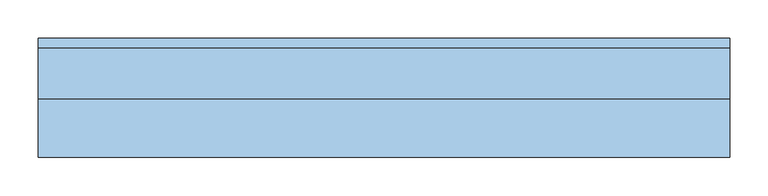
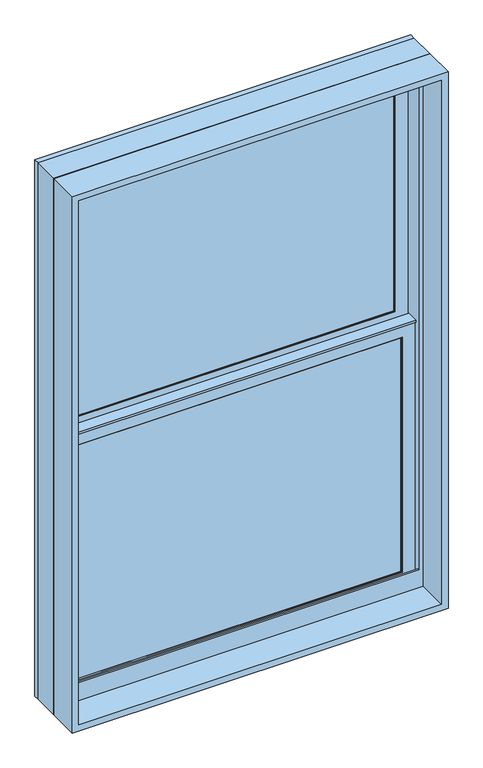
"""IFC4 building model written with IfcOpenShell, lengths in millimetres: window geometry, Window-Double_Hung-Marvin-Essential : ESDH3046."""

from ifc_helpers import new_model, si_unit, frame, origin, place, context, project, spatial, polyline, outline, extrude, faceted_brep, source, transform, mapped, element, save


def window_b4728585(model_context):
    return source(origin(), model_context, "Body", "SolidModel", [
        extrude(outline(polyline([(140.7583333, 20.6375), (140.7583333, 15.875), (121.7083333, 15.875), (121.7083333, 20.6375), (140.7583333, 20.6375)])), frame((0.0, 0.0, 1136.65), z_axis=(0.0, 0.0, 1.0), x_axis=(1.0, 0.0, 0.0)), (0.0, 0.0, 1.0), 603.25),
        extrude(outline(polyline([(-121.7083333, 20.6375), (-121.7083333, 15.875), (-140.7583333, 15.875), (-140.7583333, 20.6375), (-121.7083333, 20.6375)])), frame((0.0, 0.0, 1136.65), z_axis=(0.0, 0.0, 1.0), x_axis=(1.0, 0.0, 0.0)), (0.0, 0.0, 1.0), 603.25),
        extrude(outline(polyline([(393.7, 20.6375), (393.7, 15.875), (-393.7, 15.875), (-393.7, 20.6375), (393.7, 20.6375)])), frame((0.0, 0.0, 1428.75), z_axis=(0.0, 0.0, 1.0), x_axis=(1.0, 0.0, 0.0)), (0.0, 0.0, 1.0), 19.05),
        extrude(outline(polyline([(-140.7583333, 46.83125), (-140.7583333, 51.59375), (-121.7083333, 51.59375), (-121.7083333, 46.83125), (-140.7583333, 46.83125)])), frame((0.0, 0.0, 1778.0), z_axis=(0.0, 0.0, 1.0), x_axis=(1.0, 0.0, 0.0)), (0.0, 0.0, 1.0), 603.25),
        extrude(outline(polyline([(121.7083333, 46.83125), (121.7083333, 51.59375), (140.7583333, 51.59375), (140.7583333, 46.83125), (121.7083333, 46.83125)])), frame((0.0, 0.0, 1778.0), z_axis=(0.0, 0.0, 1.0), x_axis=(1.0, 0.0, 0.0)), (0.0, 0.0, 1.0), 603.25),
        extrude(outline(polyline([(-393.7, 46.83125), (-393.7, 51.59375), (393.7, 51.59375), (393.7, 46.83125), (-393.7, 46.83125)])), frame((0.0, 0.0, 2070.1), z_axis=(0.0, 0.0, 1.0), x_axis=(1.0, 0.0, 0.0)), (0.0, 0.0, 1.0), 19.05),
        extrude(outline(polyline([(140.7583333, 20.6375), (121.7083333, 20.6375), (121.7083333, 25.4), (140.7583333, 25.4), (140.7583333, 20.6375)])), frame((0.0, 0.0, 1136.65), z_axis=(0.0, 0.0, 1.0), x_axis=(1.0, 0.0, 0.0)), (0.0, 0.0, 1.0), 603.25),
        extrude(outline(polyline([(-121.7083333, 20.6375), (-140.7583333, 20.6375), (-140.7583333, 25.4), (-121.7083333, 25.4), (-121.7083333, 20.6375)])), frame((0.0, 0.0, 1136.65), z_axis=(0.0, 0.0, 1.0), x_axis=(1.0, 0.0, 0.0)), (0.0, 0.0, 1.0), 603.25),
        extrude(outline(polyline([(393.7, 20.6375), (-393.7, 20.6375), (-393.7, 25.4), (393.7, 25.4), (393.7, 20.6375)])), frame((0.0, 0.0, 1428.75), z_axis=(0.0, 0.0, 1.0), x_axis=(1.0, 0.0, 0.0)), (0.0, 0.0, 1.0), 19.05),
        extrude(outline(polyline([(-140.7583333, 56.35625), (-121.7083333, 56.35625), (-121.7083333, 51.59375), (-140.7583333, 51.59375), (-140.7583333, 56.35625)])), frame((0.0, 0.0, 1778.0), z_axis=(0.0, 0.0, 1.0), x_axis=(1.0, 0.0, 0.0)), (0.0, 0.0, 1.0), 603.25),
        extrude(outline(polyline([(121.7083333, 56.35625), (140.7583333, 56.35625), (140.7583333, 51.59375), (121.7083333, 51.59375), (121.7083333, 56.35625)])), frame((0.0, 0.0, 1778.0), z_axis=(0.0, 0.0, 1.0), x_axis=(1.0, 0.0, 0.0)), (0.0, 0.0, 1.0), 603.25),
        extrude(outline(polyline([(-393.7, 56.35625), (393.7, 56.35625), (393.7, 51.59375), (-393.7, 51.59375), (-393.7, 56.35625)])), frame((0.0, 0.0, 2070.1), z_axis=(0.0, 0.0, 1.0), x_axis=(1.0, 0.0, 0.0)), (0.0, 0.0, 1.0), 19.05),
        faceted_brep([(-420.6875, 5.6780605, 1769.9351748), (-420.6875, 5.6780605, 1765.3), (420.6875, 5.6780605, 1765.3), (420.6875, 5.6780605, 1769.9351748), (-420.6875, 34.8118605, 1769.9351748), (420.6875, 34.8118605, 1769.9351748), (420.6875, 34.8118605, 1765.3), (-420.6875, 34.8118605, 1765.3), (-420.6875, 30.1625, 1765.3), (-420.6875, 30.1625, 1109.6625), (-420.6875, 8.9241104, 1109.6625), (-420.6875, 8.9241104, 1765.3), (420.6875, 8.9241104, 1765.3), (420.6875, 30.1625, 1765.3), (420.6875, 8.9241104, 1109.6625), (420.6875, 30.1625, 1109.6625), (-404.8034752, 11.90625, 1751.0034752), (-404.8034752, 30.1625, 1751.0034752), (404.8034752, 30.1625, 1751.0034752), (404.8034752, 11.90625, 1751.0034752), (-388.14375, 10.4662439, 1734.34375), (-388.14375, 11.90625, 1734.34375), (388.14375, 11.90625, 1734.34375), (388.14375, 10.4662439, 1734.34375), (389.6858834, 8.9241104, 1735.8858834), (-389.6858834, 8.9241104, 1735.8858834), (404.8034752, 30.1625, 1125.5465248), (404.8034752, 11.90625, 1125.5465248), (388.14375, 11.90625, 1142.20625), (388.14375, 10.4662439, 1142.20625), (389.6858834, 8.9241104, 1140.6641166), (-404.8034752, 30.1625, 1125.5465248), (-404.8034752, 11.90625, 1125.5465248), (-388.14375, 11.90625, 1142.20625), (-388.14375, 10.4662439, 1142.20625), (-389.6858834, 8.9241104, 1140.6641166)], [[[0, 1, 2, 3]], [[4, 5, 6, 7]], [[1, 0, 4, 7, 8, 9, 10, 11]], [[2, 1, 11, 12]], [[7, 6, 13, 8]], [[3, 2, 12, 14, 15, 13, 6, 5]], [[0, 3, 5, 4]], [[16, 17, 18, 19]], [[20, 21, 22, 23]], [[20, 23, 24, 25]], [[19, 18, 26, 27]], [[23, 22, 28, 29]], [[24, 23, 29, 30]], [[27, 26, 31, 32]], [[29, 28, 33, 34]], [[30, 29, 34, 35]], [[15, 14, 10, 9]], [[15, 9, 8, 13], [18, 17, 31, 26]], [[17, 16, 32, 31]], [[16, 19, 27, 32], [22, 21, 33, 28]], [[21, 20, 34, 33]], [[20, 25, 35, 34]], [[10, 14, 12, 11], [25, 24, 30, 35]]]),
        extrude(outline(polyline([(38.5955581, 1751.0125), (33.5778968, 1751.0125), (33.5778968, 1752.6), (39.9405976, 1752.6), (39.9405976, 1751.0125), (61.515625, 1751.0125), (47.6307501, 1747.6975159), (38.5955581, 1747.6975159), (38.5955581, 1751.0125)])), frame((-420.6875, 0.0, 0.0), z_axis=(1.0, 0.0, 0.0), x_axis=(0.0, 1.0, 0.0)), (0.0, 0.0, 1.0), 841.375),
        faceted_brep([(450.85, 0.0, 1079.5), (450.85, 0.0, 2438.4), (-450.85, 0.0, 2438.4), (-450.85, 0.0, 1079.5), (424.65625, 0.0, 1140.61875), (-424.65625, 0.0, 1140.61875), (-424.65625, 0.0, 2412.20625), (424.65625, 0.0, 2412.20625), (424.65625, 3.96875, 1079.5), (-424.65625, 3.96875, 1079.5), (-424.65625, 3.96875, 1140.61875), (424.65625, 3.96875, 1140.61875), (-450.85, 65.6828125, 1079.5), (-424.65625, 65.6828125, 1079.5), (424.65625, 65.6828125, 1079.5), (450.85, 65.6828125, 1079.5), (-450.85, 65.6828125, 2438.4), (450.85, 65.6828125, 2438.4), (424.65625, 65.6828125, 2412.20625), (-424.65625, 65.6828125, 2412.20625)], [[[0, 1, 2, 3], [4, 5, 6, 7]], [[8, 9, 10, 11]], [[5, 4, 11, 10]], [[0, 3, 12, 13, 9, 8, 14, 15]], [[13, 12, 16, 17, 15, 14, 18, 19]], [[13, 19, 6, 5, 10, 9]], [[7, 6, 19, 18]], [[18, 14, 8, 11, 4, 7]], [[1, 0, 15, 17]], [[2, 1, 17, 16]], [[3, 2, 16, 12]]]),
        faceted_brep([(424.65625, 30.1625, 1758.95), (423.06875, 30.1625, 1758.95), (423.06875, 30.1625, 1103.8544613), (424.65625, 30.1625, 1103.8544613), (-423.06875, 30.1625, 1758.95), (-424.65625, 30.1625, 1758.95), (-424.65625, 30.1625, 1103.8544613), (-423.06875, 30.1625, 1103.8544613), (423.06875, 63.5, 1758.95), (424.65625, 63.5, 1758.95), (424.65625, 63.5, 1097.3743077), (423.06875, 63.5, 1097.3743077), (-424.65625, 63.5, 1758.95), (-423.06875, 63.5, 1758.95), (-423.06875, 63.5, 1097.3743077), (-424.65625, 63.5, 1097.3743077), (435.9108932, 3.96875, 1108.9460105), (435.9108932, 3.96875, 1079.5), (435.9108932, 65.6828125, 1079.5), (435.9108932, 65.6828125, 1096.950012), (-435.9108932, 3.96875, 1079.5), (-435.9108932, 3.96875, 1108.9460105), (-435.9108932, 65.6828125, 1096.950012), (-435.9108932, 65.6828125, 1079.5), (435.9108932, 78.58125, 1094.4428097), (-435.9108932, 78.58125, 1094.4428097), (-433.8971252, 68.2348864, 1096.4539391), (-415.93135, 68.2348864, 1096.4539391), (-415.93135, 65.6828125, 1096.950012), (415.93135, 65.6828125, 1096.950012), (415.93135, 68.2348864, 1096.4539391), (433.8971252, 68.2348864, 1096.4539391), (-450.85, 65.6828125, 1079.5), (-450.85, 78.5948249, 1079.5), (450.85, 78.5948249, 1079.5), (450.85, 65.6828125, 1079.5), (-450.85, 78.58125, 2438.4), (450.85, 78.58125, 2438.4), (435.9108932, 78.58125, 2423.4608932), (-435.9108932, 78.58125, 2423.4608932), (-450.85, 65.6828125, 2438.4), (-433.8971252, 68.2348864, 2421.4471252), (433.8971252, 68.2348864, 2421.4471252), (415.93135, 68.2348864, 2403.48135), (-415.93135, 68.2348864, 2403.48135), (-415.93135, 65.6828125, 2403.48135), (415.93135, 65.6828125, 2403.48135), (450.85, 65.6828125, 2438.4)], [[[0, 1, 2, 3]], [[4, 5, 6, 7]], [[8, 9, 10, 11]], [[12, 13, 14, 15]], [[1, 8, 11, 2]], [[9, 0, 3, 10]], [[1, 0, 9, 8]], [[5, 4, 13, 12]], [[5, 12, 15, 6]], [[13, 4, 7, 14]], [[16, 17, 18, 19]], [[20, 21, 22, 23]], [[24, 25, 26, 27, 28, 22, 21, 16, 19, 29, 30, 31], [3, 2, 11, 10], [7, 6, 15, 14]], [[17, 16, 21, 20]], [[17, 20, 23, 32, 33, 34, 35, 18]], [[34, 33, 36, 37], [25, 24, 38, 39]], [[33, 32, 40, 36]], [[39, 41, 26, 25]], [[41, 42, 31, 30, 43, 44, 27, 26]], [[44, 45, 28, 27]], [[40, 32, 23, 22, 28, 45, 46, 29, 19, 18, 35, 47]], [[36, 40, 47, 37]], [[39, 38, 42, 41]], [[44, 43, 46, 45]], [[34, 37, 47, 35]], [[42, 38, 24, 31]], [[46, 43, 30, 29]]]),
        extrude(outline(polyline([(400.84375, 11.90625), (-400.84375, 11.90625), (-400.84375, 15.08125), (400.84375, 15.08125), (400.84375, 11.90625)])), frame((0.0, 0.0, 1129.50625), z_axis=(0.0, 0.0, 1.0), x_axis=(1.0, 0.0, 0.0)), (0.0, 0.0, 1.0), 617.5375),
        extrude(outline(polyline([(400.84375, 42.8625), (-400.84375, 42.8625), (-400.84375, 46.0375), (400.84375, 46.0375), (400.84375, 42.8625)])), frame((0.0, 0.0, 1770.85625), z_axis=(0.0, 0.0, 1.0), x_axis=(1.0, 0.0, 0.0)), (0.0, 0.0, 1.0), 617.5375),
        faceted_brep([(-388.14375, 31.194477, 1734.34375), (-389.6858834, 32.7366104, 1735.8858834), (389.6858834, 32.7366104, 1735.8858834), (388.14375, 31.194477, 1734.34375), (-388.14375, 30.1625, 1734.34375), (388.14375, 30.1625, 1734.34375), (-420.6875, 32.7366104, 1766.8875), (-420.6875, 30.1625, 1766.8875), (420.6875, 30.1625, 1766.8875), (420.6875, 32.7366104, 1766.8875), (389.6858834, 32.7366104, 1140.6641166), (388.14375, 31.194477, 1142.20625), (388.14375, 30.1625, 1142.20625), (420.6875, 30.1625, 1109.6625), (420.6875, 32.7366104, 1109.6625), (-389.6858834, 32.7366104, 1140.6641166), (-388.14375, 31.194477, 1142.20625), (-388.14375, 30.1625, 1142.20625), (-420.6875, 30.1625, 1109.6625), (-420.6875, 32.7366104, 1109.6625)], [[[0, 1, 2, 3]], [[4, 0, 3, 5]], [[6, 7, 8, 9]], [[3, 2, 10, 11]], [[5, 3, 11, 12]], [[9, 8, 13, 14]], [[11, 10, 15, 16]], [[12, 11, 16, 17]], [[14, 13, 18, 19]], [[9, 14, 19, 6], [1, 15, 10, 2]], [[16, 15, 1, 0]], [[17, 16, 0, 4]], [[7, 18, 13, 8], [5, 12, 17, 4]], [[19, 18, 7, 6]]]),
        faceted_brep([(-404.8034752, 42.8625, 2392.3534752), (-404.8034752, 61.11875, 2392.3534752), (404.8034752, 61.11875, 2392.3534752), (404.8034752, 42.8625, 2392.3534752), (-388.14375, 41.4224939, 2375.69375), (-388.14375, 42.8625, 2375.69375), (388.14375, 42.8625, 2375.69375), (388.14375, 41.4224939, 2375.69375), (-389.6858834, 39.8803604, 2377.2358834), (389.6858834, 39.8803604, 2377.2358834), (-420.6875, 61.11875, 2408.2375), (-420.6875, 39.8803604, 2408.2375), (420.6875, 39.8803604, 2408.2375), (420.6875, 61.11875, 2408.2375), (404.8034752, 61.11875, 1766.8965248), (404.8034752, 42.8625, 1766.8965248), (388.14375, 42.8625, 1783.55625), (388.14375, 41.4224939, 1783.55625), (389.6858834, 39.8803604, 1782.0141166), (420.6875, 39.8803604, 1751.0125), (420.6875, 61.11875, 1751.0125), (-404.8034752, 61.11875, 1766.8965248), (-404.8034752, 42.8625, 1766.8965248), (-388.14375, 42.8625, 1783.55625), (-388.14375, 41.4224939, 1783.55625), (-389.6858834, 39.8803604, 1782.0141166), (-420.6875, 39.8803604, 1751.0125), (-420.6875, 61.11875, 1751.0125)], [[[0, 1, 2, 3]], [[4, 5, 6, 7]], [[8, 4, 7, 9]], [[10, 11, 12, 13]], [[3, 2, 14, 15]], [[7, 6, 16, 17]], [[9, 7, 17, 18]], [[13, 12, 19, 20]], [[15, 14, 21, 22]], [[17, 16, 23, 24]], [[18, 17, 24, 25]], [[20, 19, 26, 27]], [[13, 20, 27, 10], [1, 21, 14, 2]], [[22, 21, 1, 0]], [[3, 15, 22, 0], [5, 23, 16, 6]], [[24, 23, 5, 4]], [[25, 24, 4, 8]], [[11, 26, 19, 12], [9, 18, 25, 8]], [[27, 26, 11, 10]]]),
        faceted_brep([(-420.6875, 61.11875, 1751.0125), (-420.6875, 63.6928604, 1751.0125), (420.6875, 63.6928604, 1751.0125), (420.6875, 61.11875, 1751.0125), (-388.14375, 62.150727, 1783.55625), (-388.14375, 61.11875, 1783.55625), (388.14375, 61.11875, 1783.55625), (388.14375, 62.150727, 1783.55625), (-389.6858834, 63.6928604, 1782.0141166), (389.6858834, 63.6928604, 1782.0141166), (420.6875, 63.6928604, 2408.2375), (420.6875, 61.11875, 2408.2375), (388.14375, 61.11875, 2375.69375), (388.14375, 62.150727, 2375.69375), (389.6858834, 63.6928604, 2377.2358834), (-420.6875, 63.6928604, 2408.2375), (-420.6875, 61.11875, 2408.2375), (-388.14375, 61.11875, 2375.69375), (-388.14375, 62.150727, 2375.69375), (-389.6858834, 63.6928604, 2377.2358834)], [[[0, 1, 2, 3]], [[4, 5, 6, 7]], [[8, 4, 7, 9]], [[3, 2, 10, 11]], [[7, 6, 12, 13]], [[9, 7, 13, 14]], [[11, 10, 15, 16]], [[13, 12, 17, 18]], [[14, 13, 18, 19]], [[16, 15, 1, 0]], [[3, 11, 16, 0], [5, 17, 12, 6]], [[18, 17, 5, 4]], [[19, 18, 4, 8]], [[1, 15, 10, 2], [9, 14, 19, 8]]]),
        extrude(outline(polyline([(400.84375, 26.19375), (-400.84375, 26.19375), (-400.84375, 30.1625), (400.84375, 30.1625), (400.84375, 26.19375)])), frame((0.0, 0.0, 1129.50625), z_axis=(0.0, 0.0, 1.0), x_axis=(1.0, 0.0, 0.0)), (0.0, 0.0, 1.0), 617.5375),
        extrude(outline(polyline([(400.84375, 57.15), (-400.84375, 57.15), (-400.84375, 61.11875), (400.84375, 61.11875), (400.84375, 57.15)])), frame((0.0, 0.0, 1770.85625), z_axis=(0.0, 0.0, 1.0), x_axis=(1.0, 0.0, 0.0)), (0.0, 0.0, 1.0), 617.5375),
        extrude(outline(polyline([(2438.4, 450.85), (2438.4, -450.85), (1079.5, -450.85), (1079.5, 450.85), (2438.4, 450.85)]), holes=[polyline([(2422.525, 434.975), (1095.375, 434.975), (1095.375, -434.975), (2422.525, -434.975), (2422.525, 434.975)])]), frame((0.0, -76.2, 0.0), z_axis=(0.0, 1.0, 0.0), x_axis=(0.0, 0.0, 1.0)), (0.0, 0.0, 1.0), 75.40625),
    ])


if __name__ == "__main__":
    model = new_model("IFC4")
    model_context = context("Model", 3, world=origin())
    ifc_project = project(units=[si_unit("LENGTHUNIT", "METRE", prefix="MILLI")], contexts=[model_context])
    site = spatial("IfcSite", under=ifc_project)
    building = spatial("IfcBuilding", under=site)
    placement = place(None, origin())
    window_shape = window_b4728585(model_context)
    element("IfcWindow", 1, ObjectType="Window-Double_Hung-Marvin-Essential : ESDH3046", at=placement, inside=building, context=model_context, shape_type="MappedRepresentation", body=[
        mapped(window_shape, transform((0.0, 0.0, 0.0), x_axis=(1.0, 0.0, 0.0), y_axis=(0.0, 1.0, 0.0), z_axis=(0.0, 0.0, 1.0))),
    ])
    save(model, "model.ifc")

# Revit data of these elements
# Type "Window-Double_Hung-Marvin-Essential : ESDH3046"
#   Type Mark = "58"
#   Window Type = "Essential Double Hung"
#   Product data url = "https://bimobject.com/marvin-windows-and-doors/product/marvin-dhwau"
#   Product Guid = "c4a96547-874c-4385-91dc-a058adc19d98"
#   Frame = "All Ultrex"
#   Egress Window = "No"
#   URL = "www.marvin.com"
#   Model = "ESDH3046"
#   Manufacturer = "Marvin Windows and Doors"
#   Label Egress = ""
#   Glass Type = "IG Low E II with Argon"
#   Design Pressure = "DP50"
#   Description = "3654 DBHG"
#   Analytic Construction = "<None>"
#   Prairie Corner Width = 0' - 4"
#   Prairie Corner Height = 0' - 4"
#   Egress Width = 2' - 8 9/16"
#   Egress Height = 1' - 10 27/128"
#   Rough Width = 3' - 0"
#   Rough Height = 4' - 6"
#   Nominal Width = 3' - 0"
#   Nominal Height = 4' - 6"
#   Inset to Installation Flange [instance default] = 0' - 1"
#   Height = 4' - 5 1/2"
#   Egress Area = 5.02253 SF
#   Default Head Height = 8' - 0"
#   Width = 2' - 11 1/2"
#   Daylight Area = 9.89567 SF
#   DLO Width = 2' - 6 9/16"
#   DLO Height = 1' - 11 5/16"
#   Muntins Top Sash = yes
#   Lites Wide Top Sash = 3
#   Lites Wide Bottom Sash = 3
#   Lites High Top Sash = 2
#   Lites High Bottom Sash = 2
#   Lite Cut Prairie 9 = no
#   Lite Cut HV Grid = yes
#   Muntins Bottom Sash = yes
#   Label Visibility = no
#   Jamb Extension Visibility = yes
#   Edition number = 1
#   Interior Material = Ultrex-Marvin-Stonewhite
#   Glazing Material = Glass-Marvin-IG Low E II with Argon
#   Cladding Material = Ultrex-Marvin-Pebblegray
#   Wall Closure = (empty or 0)
#   Assembly Code = ""
# Element 1 (IfcWindow, "Window-Double_Hung-Marvin-Essential : ESDH3046")
#   Materials on its faces: "Ultrex-Marvin-Pebblegray", "Ultrex-Marvin-Stonewhite", "Glass-Marvin-IG Low E II with Argon"
# Materials
#   "Ultrex-Marvin-Stonewhite": class "Paint", colour RGB 250 251 245, transparency 0
#   "Glass-Marvin-IG Low E II with Argon": class "Glass", colour RGB 0 128 192, transparency 0.85
#   "Ultrex-Marvin-Pebblegray": class "Paint", colour RGB 189 185 173, transparency 0
